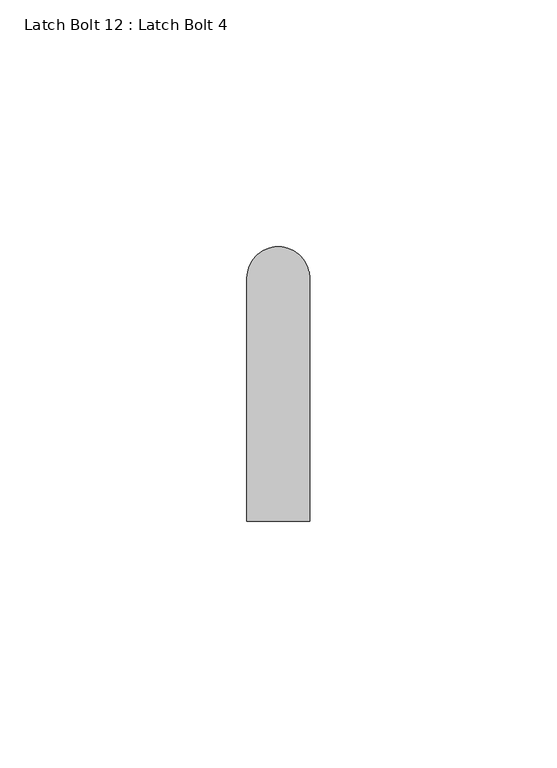
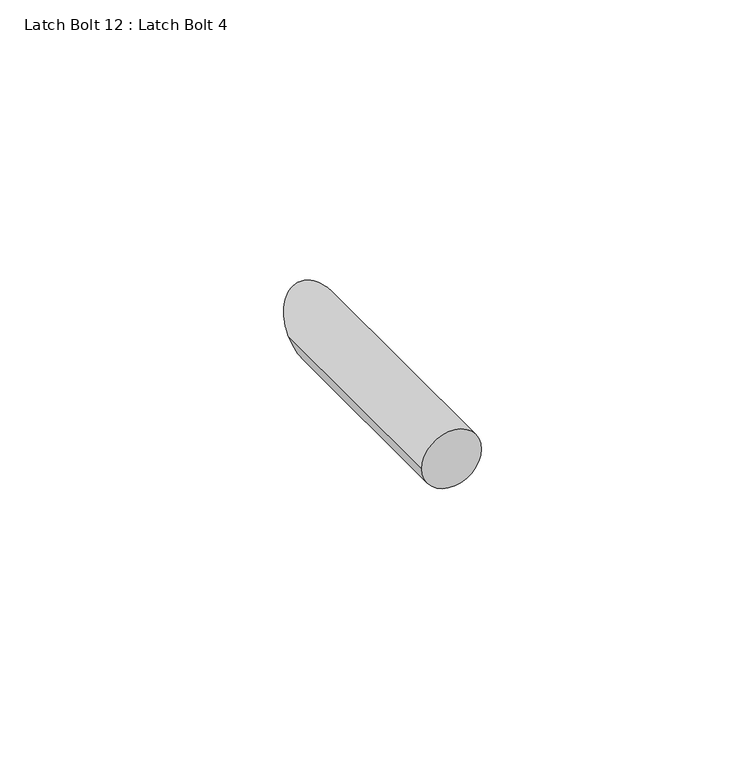
"""IFC4 building model written with IfcOpenShell, lengths in millimetres: proxy geometry, Latch Bolt 12 : Latch Bolt 4."""

from ifc_helpers import new_model, si_unit, frame, origin, place, context, project, spatial, circle_curve, ellipse_curve, source, transform, mapped, element, save
from ifc_brep_helpers import plane_surface, cylinder_surface, advanced_brep


def latch_bolt_12_latch_bolt_4_94dad4aa(model_context):
    return source(origin(), model_context, "Body", "AdvancedBrep", [
        advanced_brep(
        [(587315.8935739, -532888.5610985, 292.1), (587303.1935739, -532888.5610985, 292.1), (587315.8935739, -532839.3485985, 292.1), (587303.1935739, -532839.3485985, 292.1)],
        [
            (0, 1, circle_curve(frame((587309.5435739, -532888.5610985, 292.1), z_axis=(0.0, -1.0, 0.0), x_axis=(1.0, 0.0, 0.0)), 6.35)),
            (1, 0, circle_curve(frame((587309.5435739, -532888.5610985, 292.1), z_axis=(0.0, -1.0, 0.0), x_axis=(1.0, 0.0, 0.0)), 6.35)),
            (0, 2),
            (2, 3, ellipse_curve(frame((587309.5435739, -532839.3485985, 292.1), z_axis=(0.0, -0.7071067811865497, 0.7071067811865455), x_axis=(0.0, -0.7071067811865454, -0.7071067811865497)), 8.9802561, 6.35)),
            (3, 1),
            (3, 2, ellipse_curve(frame((587309.5435739, -532839.3485985, 292.1), z_axis=(0.0, -0.7071067811865497, 0.7071067811865455), x_axis=(0.0, -0.7071067811865454, -0.7071067811865497)), 8.9802561, 6.35)),
        ],
        [
            plane_surface(frame((587315.8935739, -532888.5610985, 292.1), z_axis=(0.0, -1.0, 0.0), x_axis=(0.0, 0.0, 1.0))),
            cylinder_surface(frame((587309.5435739, -532831.4110985, 292.1), z_axis=(0.0, -1.0, 0.0), x_axis=(1.0, 0.0, 0.0)), 6.35),
            plane_surface(frame((587338.1185739, -532847.2860985, 284.1625), z_axis=(0.0, 0.7071067811865497, -0.7071067811865455), x_axis=(-1.0, 0.0, 0.0))),
        ],
        [
            (0, [[1, 2]]),
            (1, [[-1, 3, 4, 5]]),
            (1, [[-2, -5, 6, -3]]),
            (2, [[-4, -6]]),
        ],
    ),
    ])


if __name__ == "__main__":
    model = new_model("IFC4")
    model_context = context("Model", 3, world=origin())
    ifc_project = project(units=[si_unit("LENGTHUNIT", "METRE", prefix="MILLI")], contexts=[model_context])
    site = spatial("IfcSite", under=ifc_project)
    building = spatial("IfcBuilding", under=site)
    placement = place(None, origin())
    latch_bolt_12_latch_bolt_4_shape = latch_bolt_12_latch_bolt_4_94dad4aa(model_context)
    element("IfcBuildingElementProxy", 1, Name="Latch Bolt 12 : Latch Bolt 4", ObjectType="Latch Bolt 12 : Latch Bolt 4", at=placement, inside=building, context=model_context, shape_type="MappedRepresentation", body=[
        mapped(latch_bolt_12_latch_bolt_4_shape, transform((0.0, 0.0, 0.0), x_axis=(1.0, 0.0, 0.0), y_axis=(0.0, 1.0, 0.0), z_axis=(0.0, 0.0, 1.0))),
    ])
    save(model, "model.ifc")

# Revit data of these elements
# Element 1 (IfcBuildingElementProxy, "Latch Bolt 12 : Latch Bolt 4")
#   Materials on its faces: "GALV. SLIDE BOLT"
# Materials
#   "GALV. SLIDE BOLT": class "Metal", colour RGB 189 187 185, transparency 0, Description = "Carbon steel", Cost = 0
